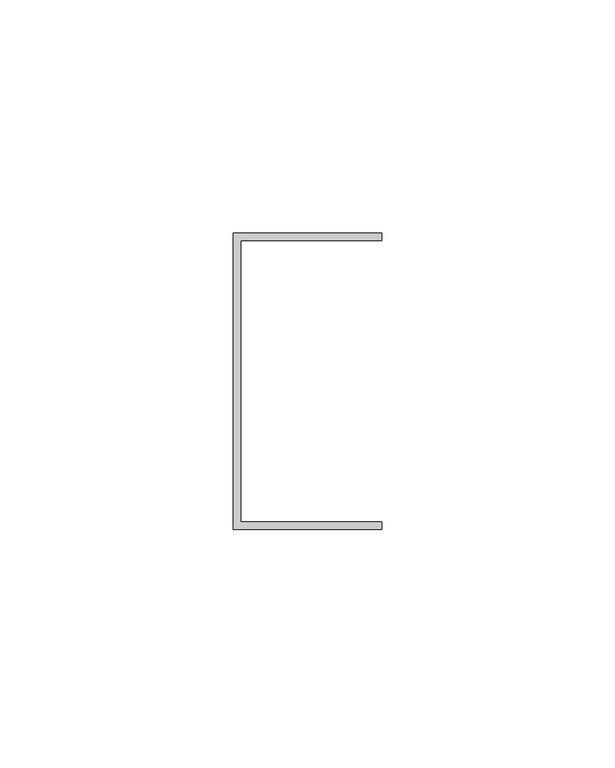
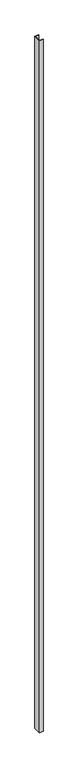
"""IFC4 building model written with IfcOpenShell, lengths in millimetres: proxy geometry, Generic Models 7:Generic Models 1:3:Generic Models 1:3 : Generic Models 7:Generic Models 1:305549:3:Generic Models 1:3:Generic Models 1:3 : Generic Models 7:Generic Models 1:305549:3 : Generic Models 7:Generic Models 1:3:Generic Models 1:3 : Generic Models 7:Generic Models 1:305549:301244:46 : Generic Models 7:Generic Models 1:3:Generic Models 1:3 : Generic Models 7:Generic Models 1:305549:3:Generic Models 1:3:Generic Models 1:3 : Generic Models 7:Generic Models 1:305549:3 : Generic Models 7:Generic Models 1:3:Generic Models 1:3 : Generic Models 7:Generic Models 1:305549:301244:308848."""

from ifc_helpers import new_model, si_unit, origin, origin_with_axes, place, context, project, spatial, polyline, outline, extrude, source, transform, mapped, element, save


def generic_models_ffa93498(model_context):
    return source(origin(), model_context, "Body", "SweptSolid", [
        extrude(outline(polyline([(803177.9632437, -579013.3913841), (803209.7132437, -579013.3913841), (803209.7132437, -579014.9788841), (803179.5507437, -579014.9788841), (803179.5507437, -579075.3038841), (803209.7132437, -579075.3038841), (803209.7132437, -579076.8913841), (803177.9632437, -579076.8913841), (803177.9632437, -579013.3913841)])), origin_with_axes(), (0.0, 0.0, 1.0), 6134.1),
    ])


if __name__ == "__main__":
    model = new_model("IFC4")
    model_context = context("Model", 3, world=origin())
    ifc_project = project(units=[si_unit("LENGTHUNIT", "METRE", prefix="MILLI")], contexts=[model_context])
    site = spatial("IfcSite", under=ifc_project)
    building = spatial("IfcBuilding", under=site)
    placement = place(None, origin())
    generic_models_shape = generic_models_ffa93498(model_context)
    element("IfcBuildingElementProxy", 1, Name="Generic Models 7:Generic Models 1:3:Generic Models 1:3 : Generic Models 7:Generic Models 1:305549:3:Generic Models 1:3:Generic Models 1:3 : Generic Models 7:Generic Models 1:305549:3 : Generic Models 7:Generic Models 1:3:Generic Models 1:3 : Generic Models 7:Generic Models 1:305549:301244:46 : Generic Models 7:Generic Models 1:3:Generic Models 1:3 : Generic Models 7:Generic Models 1:305549:3:Generic Models 1:3:Generic Models 1:3 : Generic Models 7:Generic Models 1:305549:3 : Generic Models 7:Generic Models 1:3:Generic Models 1:3 : Generic Models 7:Generic Models 1:305549:301244:308848", ObjectType="Generic Models 7:Generic Models 1:3:Generic Models 1:3 : Generic Models 7:Generic Models 1:305549:3:Generic Models 1:3:Generic Models 1:3 : Generic Models 7:Generic Models 1:305549:3 : Generic Models 7:Generic Models 1:3:Generic Models 1:3 : Generic Models 7:Generic Models 1:305549:301244:46 : Generic Models 7:Generic Models 1:3:Generic Models 1:3 : Generic Models 7:Generic Models 1:305549:3:Generic Models 1:3:Generic Models 1:3 : Generic Models 7:Generic Models 1:305549:3 : Generic Models 7:Generic Models 1:3:Generic Models 1:3 : Generic Models 7:Generic Models 1:305549:301244:308848", at=placement, inside=building, context=model_context, shape_type="MappedRepresentation", body=[
        mapped(generic_models_shape, transform((0.0, 0.0, 0.0), x_axis=(1.0, 0.0, 0.0), y_axis=(0.0, 1.0, 0.0), z_axis=(0.0, 0.0, 1.0))),
    ])
    save(model, "model.ifc")

# Revit data of these elements
# Type "Generic Models 7:Generic Models 1:3:Generic Models 1:3 : Generic Models 7:Generic Models 1:305549:3:Generic Models 1:3:Generic Models 1:3 : Generic Models 7:Generic Models 1:305549:3 : Generic Models 7:Generic Models 1:3:Generic Models 1:3 : Generic Models 7:Generic Models 1:305549:301244:46 : Generic Models 7:Generic Models 1:3:Generic Models 1:3 : Generic Models 7:Generic Models 1:305549:3:Generic Models 1:3:Generic Models 1:3 : Generic Models 7:Generic Models 1:305549:3 : Generic Models 7:Generic Models 1:3:Generic Models 1:3 : Generic Models 7:Generic Models 1:305549:301244:308848"
#   NameOverride = "Generic Models 7:Generic Models 1:3:Generic Models 1:3 : Generic Models 7:Generic Models 1:305549:3:Generic Models 1:3:Generic Models 1:3 : Generic Models 7:Generic Models 1:305549:3 : Generic Models 7:Generic Models 1:3:Generic Models 1:3 : Generic Models 7:Generic Models 1:305549:301244:308848"
#   ObjectTypeOverride = "Generic Models 1:3:Generic Models 1:3 : Generic Models 7:Generic Models 1:305549:3 : Generic Models 7:Generic Models 1:3:Generic Models 1:3 : Generic Models 7:Generic Models 1:305549:301244"
#   Reference = "Generic Models 1"
#   Tag = "308848"
# Element 1 (IfcBuildingElementProxy, "Generic Models 7:Generic Models 1:3:Generic Models 1:3 : Generic Models 7:Generic Models 1:305549:3:Generic Models 1:3:Generic Models 1:3 : Generic Models 7:Generic Models 1:305549:3 : Generic Models 7:Generic Models 1:3:Generic Models 1:3 : Generic Models 7:Generic Models 1:305549:301244:46 : Generic Models 7:Generic Models 1:3:Generic Models 1:3 : Generic Models 7:Generic Models 1:305549:3:Generic Models 1:3:Generic Models 1:3 : Generic Models 7:Generic Models 1:305549:3 : Generic Models 7:Generic Models 1:3:Generic Models 1:3 : Generic Models 7:Generic Models 1:305549:301244:308848")
#   Materials on its faces: "GALVANIZED U-CHANNEL (250T125-33)"
# Materials
#   "GALVANIZED U-CHANNEL (250T125-33)": class "Unassigned", colour RGB 202 201 200, transparency 0, Keynote = "M05451300.02", Cost = 0
